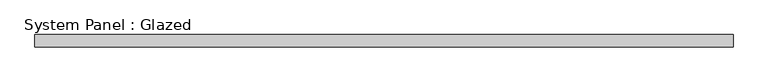
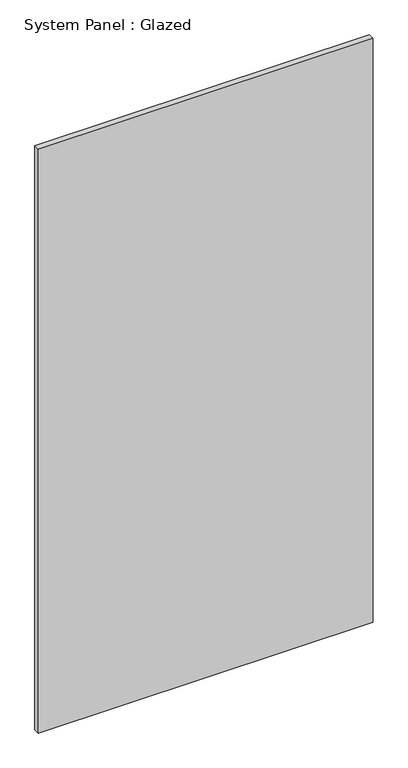
"""IFC4 building model written with IfcOpenShell, lengths in millimetres: plate geometry, System Panel : Glazed."""

from ifc_helpers import new_model, si_unit, origin, origin_with_axes, place, context, project, spatial, polyline, outline, extrude, source, transform, mapped, element, save


def system_panel_glazed_ee6efdaa(model_context):
    return source(origin(), model_context, "Body", "SweptSolid", [
        extrude(outline(polyline([(712.5, -49.5), (-712.5, -49.5), (-712.5, -24.5), (712.5, -24.5), (712.5, -49.5)])), origin_with_axes(), (0.0, 0.0, 1.0), 2625.0),
    ])


if __name__ == "__main__":
    model = new_model("IFC4")
    model_context = context("Model", 3, world=origin())
    ifc_project = project(units=[si_unit("LENGTHUNIT", "METRE", prefix="MILLI")], contexts=[model_context])
    site = spatial("IfcSite", under=ifc_project)
    building = spatial("IfcBuilding", under=site)
    placement = place(None, origin())
    system_panel_glazed_shape = system_panel_glazed_ee6efdaa(model_context)
    element("IfcPlate", 1, ObjectType="System Panel : Glazed", at=placement, inside=building, context=model_context, shape_type="MappedRepresentation", body=[
        mapped(system_panel_glazed_shape, transform((0.0, 0.0, 0.0), x_axis=(1.0, 0.0, 0.0), y_axis=(0.0, 1.0, 0.0), z_axis=(0.0, 0.0, 1.0))),
    ])
    save(model, "model.ifc")

# Revit data of these elements
# Type "System Panel : Glazed"
#   Keynote = "H11"
#   Construction Type Id = "GSP4R"
#   Analytic Construction = "1/8 in Pilkington single glazing"
#   Visual Light Transmittance = 0.9
#   Solar Heat Gain Coefficient = 0.86
#   Heat Transfer Coefficient (U) = 6.7069 W/(m²·K)
# Element 1 (IfcPlate, "System Panel : Glazed")
#   Materials on its faces: "Glass"
# Materials
#   "Glass": class "Glass", colour RGB 0 128 192, transparency 0.9, Description = "Soda Lime Glass", Cost = 0
